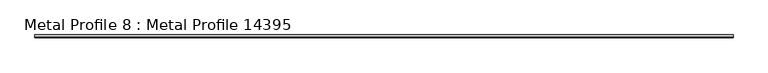
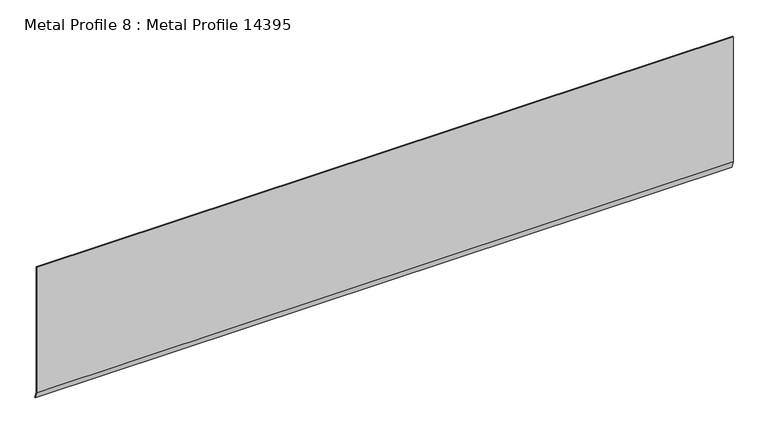
"""IFC4 building model written with IfcOpenShell, lengths in millimetres: proxy geometry, Metal Profile 8 : Metal Profile 14395."""

from ifc_helpers import new_model, si_unit, frame, origin, place, context, project, spatial, polyline, outline, extrude, source, transform, mapped, element, save


def metal_profile_8_metal_profile_14395_3c745785(model_context):
    return source(origin(), model_context, "Body", "SweptSolid", [
        extrude(outline(polyline([(10819.8958797, 43879.1077231), (10821.8958797, 43879.1077231), (10821.8958797, 43499.1077231), (10828.2608778, 43479.4565227), (10826.3581946, 43478.8402461), (10819.8958797, 43498.7919011), (10819.8958797, 43879.1077231)])), frame((3627.1904023, 0.0, 0.0), z_axis=(1.0, 0.0, 0.0), x_axis=(0.0, 1.0, 0.0)), (0.0, 0.0, 1.0), 1999.85),
    ])


if __name__ == "__main__":
    model = new_model("IFC4")
    model_context = context("Model", 3, world=origin())
    ifc_project = project(units=[si_unit("LENGTHUNIT", "METRE", prefix="MILLI")], contexts=[model_context])
    site = spatial("IfcSite", under=ifc_project)
    building = spatial("IfcBuilding", under=site)
    placement = place(None, origin())
    metal_profile_8_metal_profile_14395_shape = metal_profile_8_metal_profile_14395_3c745785(model_context)
    element("IfcBuildingElementProxy", 1, Name="Metal Profile 8 : Metal Profile 14395", ObjectType="Metal Profile 8 : Metal Profile 14395", at=placement, inside=building, context=model_context, shape_type="MappedRepresentation", body=[
        mapped(metal_profile_8_metal_profile_14395_shape, transform((0.0, 0.0, 0.0), x_axis=(1.0, 0.0, 0.0), y_axis=(0.0, 1.0, 0.0), z_axis=(0.0, 0.0, 1.0))),
    ])
    save(model, "model.ifc")

# Revit data of these elements
# Type "Metal Profile 8 : Metal Profile 14395"
#   NameOverride = "Metal Profile"
# Element 1 (IfcBuildingElementProxy, "Metal Profile 8 : Metal Profile 14395")
#   Materials on its faces: "20 GA. CONTINUOUS CLEAT"
# Materials
#   "20 GA. CONTINUOUS CLEAT": class "Unassigned", colour RGB 245 226 176, transparency 0, Cost = 0
